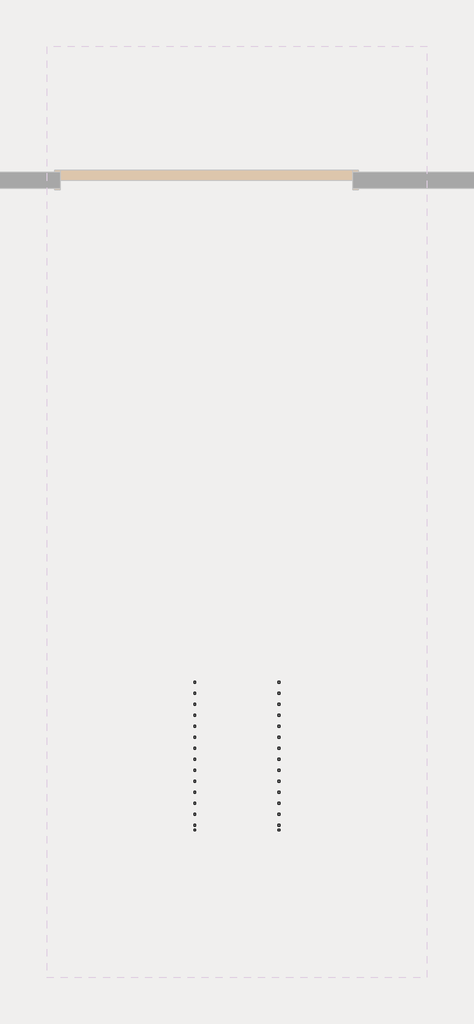
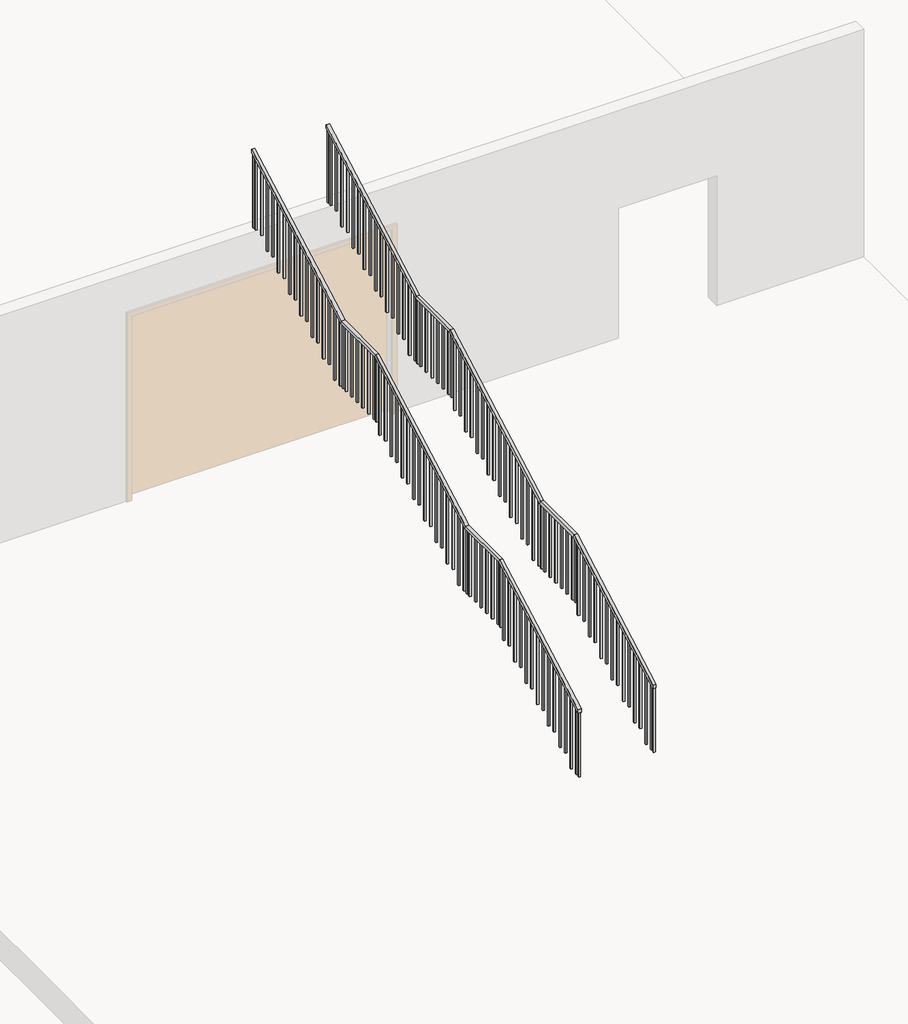
# One storey, part 9 of 13: 2 railings.
"""IFC4 building model written with IfcOpenShell, lengths in millimetres."""

from ifc_helpers import new_model, si_unit, frame, origin, place, context, project, spatial, polyline, outline, extrude, faceted_brep, element, save

model = new_model("IFC4")

# Units and contexts
model_context = context("Model", 3, world=origin())
ifc_project = project(units=[si_unit("LENGTHUNIT", "METRE", prefix="MILLI")], contexts=[model_context])

# Site, building, storey
site = spatial("IfcSite", under=ifc_project)
building = spatial("IfcBuilding", under=site)
storey = spatial("IfcBuildingStorey", under=building, Name="L0 - Ground Floor (Shadows On)", Elevation=0.0)

# Railings
placement = place(None, origin())
element("IfcRailing", 1, ObjectType="1100mm", at=placement, inside=storey, context=model_context, shape_type="SolidModel", body=[
    faceted_brep([(20443.6510627, -13941.7341454, 1266.6666667), (20443.6510627, -13941.7341454, 1209.4687214), (20493.6510627, -13941.7341454, 1209.4687214), (20493.6510627, -13941.7341454, 1266.6666667), (20443.6510627, -11841.7341454, 2433.3333333), (20443.6510627, -11828.7778439, 2383.3333333), (20493.6510627, -11828.7778439, 2383.3333333), (20493.6510627, -11841.7341454, 2433.3333333), (20443.6510627, -10941.7341454, 2433.3333333), (20443.6510627, -10928.7778439, 2383.3333333), (20493.6510627, -10928.7778439, 2383.3333333), (20493.6510627, -10941.7341454, 2433.3333333), (20443.6510627, -8541.7341454, 3766.6666667), (20443.6510627, -8528.7778439, 3716.6666667), (20493.6510627, -8528.7778439, 3716.6666667), (20493.6510627, -8541.7341454, 3766.6666667), (20443.6510627, -7641.7341454, 3766.6666667), (20443.6510627, -7628.7778439, 3716.6666667), (20493.6510627, -7628.7778439, 3716.6666667), (20493.6510627, -7641.7341454, 3766.6666667), (20443.6510627, -5241.7341454, 5100.0), (20493.6510627, -5241.7341454, 5100.0), (20493.6510627, -5241.7341454, 5042.8020548), (20443.6510627, -5241.7341454, 5042.8020548)], [[[0, 1, 2, 3]], [[1, 0, 4, 5]], [[2, 1, 5, 6]], [[3, 2, 6, 7]], [[0, 3, 7, 4]], [[5, 4, 8, 9]], [[6, 5, 9, 10]], [[7, 6, 10, 11]], [[4, 7, 11, 8]], [[9, 8, 12, 13]], [[10, 9, 13, 14]], [[11, 10, 14, 15]], [[8, 11, 15, 12]], [[13, 12, 16, 17]], [[14, 13, 17, 18]], [[15, 14, 18, 19]], [[12, 15, 19, 16]], [[20, 21, 22, 23]], [[17, 16, 20, 23]], [[18, 17, 23, 22]], [[19, 18, 22, 21]], [[16, 19, 21, 20]]]),
    extrude(outline(polyline([(-5329.2341454, 3833.3333333), (-5329.2341454, 4994.1909437), (-5304.2341454, 5008.0798326), (-5304.2341454, 3833.3333333), (-5329.2341454, 3833.3333333)])), frame((20456.1510627, 0.0, 0.0), z_axis=(1.0, 0.0, 0.0), x_axis=(0.0, 1.0, 0.0)), (0.0, 0.0, 1.0), 25.0),
    extrude(outline(polyline([(-5479.2341454, 3833.3333333), (-5479.2341454, 4910.8576103), (-5454.2341454, 4924.7464992), (-5454.2341454, 3833.3333333), (-5479.2341454, 3833.3333333)])), frame((20456.1510627, 0.0, 0.0), z_axis=(1.0, 0.0, 0.0), x_axis=(0.0, 1.0, 0.0)), (0.0, 0.0, 1.0), 25.0),
    extrude(outline(polyline([(-5629.2341454, 3666.6666667), (-5629.2341454, 4827.524277), (-5604.2341454, 4841.4131659), (-5604.2341454, 3666.6666667), (-5629.2341454, 3666.6666667)])), frame((20456.1510627, 0.0, 0.0), z_axis=(1.0, 0.0, 0.0), x_axis=(0.0, 1.0, 0.0)), (0.0, 0.0, 1.0), 25.0),
    extrude(outline(polyline([(-5779.2341454, 3666.6666667), (-5779.2341454, 4744.1909437), (-5754.2341454, 4758.0798326), (-5754.2341454, 3666.6666667), (-5779.2341454, 3666.6666667)])), frame((20456.1510627, 0.0, 0.0), z_axis=(1.0, 0.0, 0.0), x_axis=(0.0, 1.0, 0.0)), (0.0, 0.0, 1.0), 25.0),
    extrude(outline(polyline([(-5929.2341454, 3500.0), (-5929.2341454, 4660.8576103), (-5904.2341454, 4674.7464992), (-5904.2341454, 3500.0), (-5929.2341454, 3500.0)])), frame((20456.1510627, 0.0, 0.0), z_axis=(1.0, 0.0, 0.0), x_axis=(0.0, 1.0, 0.0)), (0.0, 0.0, 1.0), 25.0),
    extrude(outline(polyline([(-6079.2341454, 3500.0), (-6079.2341454, 4577.524277), (-6054.2341454, 4591.4131659), (-6054.2341454, 3500.0), (-6079.2341454, 3500.0)])), frame((20456.1510627, 0.0, 0.0), z_axis=(1.0, 0.0, 0.0), x_axis=(0.0, 1.0, 0.0)), (0.0, 0.0, 1.0), 25.0),
    extrude(outline(polyline([(-6229.2341454, 3333.3333333), (-6229.2341454, 4494.1909437), (-6204.2341454, 4508.0798326), (-6204.2341454, 3333.3333333), (-6229.2341454, 3333.3333333)])), frame((20456.1510627, 0.0, 0.0), z_axis=(1.0, 0.0, 0.0), x_axis=(0.0, 1.0, 0.0)), (0.0, 0.0, 1.0), 25.0),
    extrude(outline(polyline([(-6379.2341454, 3333.3333333), (-6379.2341454, 4410.8576103), (-6354.2341454, 4424.7464992), (-6354.2341454, 3333.3333333), (-6379.2341454, 3333.3333333)])), frame((20456.1510627, 0.0, 0.0), z_axis=(1.0, 0.0, 0.0), x_axis=(0.0, 1.0, 0.0)), (0.0, 0.0, 1.0), 25.0),
    extrude(outline(polyline([(-6529.2341454, 3166.6666667), (-6529.2341454, 4327.524277), (-6504.2341454, 4341.4131659), (-6504.2341454, 3166.6666667), (-6529.2341454, 3166.6666667)])), frame((20456.1510627, 0.0, 0.0), z_axis=(1.0, 0.0, 0.0), x_axis=(0.0, 1.0, 0.0)), (0.0, 0.0, 1.0), 25.0),
    extrude(outline(polyline([(-6679.2341454, 3166.6666667), (-6679.2341454, 4244.1909437), (-6654.2341454, 4258.0798326), (-6654.2341454, 3166.6666667), (-6679.2341454, 3166.6666667)])), frame((20456.1510627, 0.0, 0.0), z_axis=(1.0, 0.0, 0.0), x_axis=(0.0, 1.0, 0.0)), (0.0, 0.0, 1.0), 25.0),
    extrude(outline(polyline([(-6829.2341454, 3000.0), (-6829.2341454, 4160.8576103), (-6804.2341454, 4174.7464992), (-6804.2341454, 3000.0), (-6829.2341454, 3000.0)])), frame((20456.1510627, 0.0, 0.0), z_axis=(1.0, 0.0, 0.0), x_axis=(0.0, 1.0, 0.0)), (0.0, 0.0, 1.0), 25.0),
    extrude(outline(polyline([(-6979.2341454, 3000.0), (-6979.2341454, 4077.524277), (-6954.2341454, 4091.4131659), (-6954.2341454, 3000.0), (-6979.2341454, 3000.0)])), frame((20456.1510627, 0.0, 0.0), z_axis=(1.0, 0.0, 0.0), x_axis=(0.0, 1.0, 0.0)), (0.0, 0.0, 1.0), 25.0),
    extrude(outline(polyline([(-7129.2341454, 2833.3333333), (-7129.2341454, 3994.1909437), (-7104.2341454, 4008.0798326), (-7104.2341454, 2833.3333333), (-7129.2341454, 2833.3333333)])), frame((20456.1510627, 0.0, 0.0), z_axis=(1.0, 0.0, 0.0), x_axis=(0.0, 1.0, 0.0)), (0.0, 0.0, 1.0), 25.0),
    extrude(outline(polyline([(-7279.2341454, 2833.3333333), (-7279.2341454, 3910.8576103), (-7254.2341454, 3924.7464992), (-7254.2341454, 2833.3333333), (-7279.2341454, 2833.3333333)])), frame((20456.1510627, 0.0, 0.0), z_axis=(1.0, 0.0, 0.0), x_axis=(0.0, 1.0, 0.0)), (0.0, 0.0, 1.0), 25.0),
    extrude(outline(polyline([(-7429.2341454, 2666.6666667), (-7429.2341454, 3827.524277), (-7404.2341454, 3841.4131659), (-7404.2341454, 2666.6666667), (-7429.2341454, 2666.6666667)])), frame((20456.1510627, 0.0, 0.0), z_axis=(1.0, 0.0, 0.0), x_axis=(0.0, 1.0, 0.0)), (0.0, 0.0, 1.0), 25.0),
    extrude(outline(polyline([(-7579.2341454, 2666.6666667), (-7579.2341454, 3744.1909437), (-7554.2341454, 3758.0798326), (-7554.2341454, 2666.6666667), (-7579.2341454, 2666.6666667)])), frame((20456.1510627, 0.0, 0.0), z_axis=(1.0, 0.0, 0.0), x_axis=(0.0, 1.0, 0.0)), (0.0, 0.0, 1.0), 25.0),
    extrude(outline(polyline([(20481.1510627, -7729.2341454), (20456.1510627, -7729.2341454), (20456.1510627, -7704.2341454), (20481.1510627, -7704.2341454), (20481.1510627, -7729.2341454)])), frame((0.0, 0.0, 2666.6666667), z_axis=(0.0, 0.0, 1.0), x_axis=(1.0, 0.0, 0.0)), (0.0, 0.0, 1.0), 1050.0),
    extrude(outline(polyline([(20481.1510627, -7879.2341454), (20456.1510627, -7879.2341454), (20456.1510627, -7854.2341454), (20481.1510627, -7854.2341454), (20481.1510627, -7879.2341454)])), frame((0.0, 0.0, 2666.6666667), z_axis=(0.0, 0.0, 1.0), x_axis=(1.0, 0.0, 0.0)), (0.0, 0.0, 1.0), 1050.0),
    extrude(outline(polyline([(20481.1510627, -8029.2341454), (20456.1510627, -8029.2341454), (20456.1510627, -8004.2341454), (20481.1510627, -8004.2341454), (20481.1510627, -8029.2341454)])), frame((0.0, 0.0, 2666.6666667), z_axis=(0.0, 0.0, 1.0), x_axis=(1.0, 0.0, 0.0)), (0.0, 0.0, 1.0), 1050.0),
    extrude(outline(polyline([(20481.1510627, -8179.2341454), (20456.1510627, -8179.2341454), (20456.1510627, -8154.2341454), (20481.1510627, -8154.2341454), (20481.1510627, -8179.2341454)])), frame((0.0, 0.0, 2666.6666667), z_axis=(0.0, 0.0, 1.0), x_axis=(1.0, 0.0, 0.0)), (0.0, 0.0, 1.0), 1050.0),
    extrude(outline(polyline([(20481.1510627, -8329.2341454), (20456.1510627, -8329.2341454), (20456.1510627, -8304.2341454), (20481.1510627, -8304.2341454), (20481.1510627, -8329.2341454)])), frame((0.0, 0.0, 2666.6666667), z_axis=(0.0, 0.0, 1.0), x_axis=(1.0, 0.0, 0.0)), (0.0, 0.0, 1.0), 1050.0),
    extrude(outline(polyline([(20481.1510627, -8479.2341454), (20456.1510627, -8479.2341454), (20456.1510627, -8454.2341454), (20481.1510627, -8454.2341454), (20481.1510627, -8479.2341454)])), frame((0.0, 0.0, 2666.6666667), z_axis=(0.0, 0.0, 1.0), x_axis=(1.0, 0.0, 0.0)), (0.0, 0.0, 1.0), 1050.0),
    extrude(outline(polyline([(-8629.2341454, 2500.0), (-8629.2341454, 3660.8576103), (-8604.2341454, 3674.7464992), (-8604.2341454, 2500.0), (-8629.2341454, 2500.0)])), frame((20456.1510627, 0.0, 0.0), z_axis=(1.0, 0.0, 0.0), x_axis=(0.0, 1.0, 0.0)), (0.0, 0.0, 1.0), 25.0),
    extrude(outline(polyline([(-8779.2341454, 2500.0), (-8779.2341454, 3577.524277), (-8754.2341454, 3591.4131659), (-8754.2341454, 2500.0), (-8779.2341454, 2500.0)])), frame((20456.1510627, 0.0, 0.0), z_axis=(1.0, 0.0, 0.0), x_axis=(0.0, 1.0, 0.0)), (0.0, 0.0, 1.0), 25.0),
    extrude(outline(polyline([(-8929.2341454, 2333.3333333), (-8929.2341454, 3494.1909437), (-8904.2341454, 3508.0798326), (-8904.2341454, 2333.3333333), (-8929.2341454, 2333.3333333)])), frame((20456.1510627, 0.0, 0.0), z_axis=(1.0, 0.0, 0.0), x_axis=(0.0, 1.0, 0.0)), (0.0, 0.0, 1.0), 25.0),
    extrude(outline(polyline([(-9079.2341454, 2333.3333333), (-9079.2341454, 3410.8576103), (-9054.2341454, 3424.7464992), (-9054.2341454, 2333.3333333), (-9079.2341454, 2333.3333333)])), frame((20456.1510627, 0.0, 0.0), z_axis=(1.0, 0.0, 0.0), x_axis=(0.0, 1.0, 0.0)), (0.0, 0.0, 1.0), 25.0),
    extrude(outline(polyline([(-9229.2341454, 2166.6666667), (-9229.2341454, 3327.524277), (-9204.2341454, 3341.4131659), (-9204.2341454, 2166.6666667), (-9229.2341454, 2166.6666667)])), frame((20456.1510627, 0.0, 0.0), z_axis=(1.0, 0.0, 0.0), x_axis=(0.0, 1.0, 0.0)), (0.0, 0.0, 1.0), 25.0),
    extrude(outline(polyline([(-9379.2341454, 2166.6666667), (-9379.2341454, 3244.1909437), (-9354.2341454, 3258.0798326), (-9354.2341454, 2166.6666667), (-9379.2341454, 2166.6666667)])), frame((20456.1510627, 0.0, 0.0), z_axis=(1.0, 0.0, 0.0), x_axis=(0.0, 1.0, 0.0)), (0.0, 0.0, 1.0), 25.0),
    extrude(outline(polyline([(-9529.2341454, 2000.0), (-9529.2341454, 3160.8576103), (-9504.2341454, 3174.7464992), (-9504.2341454, 2000.0), (-9529.2341454, 2000.0)])), frame((20456.1510627, 0.0, 0.0), z_axis=(1.0, 0.0, 0.0), x_axis=(0.0, 1.0, 0.0)), (0.0, 0.0, 1.0), 25.0),
    extrude(outline(polyline([(-9679.2341454, 2000.0), (-9679.2341454, 3077.524277), (-9654.2341454, 3091.4131659), (-9654.2341454, 2000.0), (-9679.2341454, 2000.0)])), frame((20456.1510627, 0.0, 0.0), z_axis=(1.0, 0.0, 0.0), x_axis=(0.0, 1.0, 0.0)), (0.0, 0.0, 1.0), 25.0),
    extrude(outline(polyline([(-9829.2341454, 1833.3333333), (-9829.2341454, 2994.1909437), (-9804.2341454, 3008.0798326), (-9804.2341454, 1833.3333333), (-9829.2341454, 1833.3333333)])), frame((20456.1510627, 0.0, 0.0), z_axis=(1.0, 0.0, 0.0), x_axis=(0.0, 1.0, 0.0)), (0.0, 0.0, 1.0), 25.0),
    extrude(outline(polyline([(-9979.2341454, 1833.3333333), (-9979.2341454, 2910.8576103), (-9954.2341454, 2924.7464992), (-9954.2341454, 1833.3333333), (-9979.2341454, 1833.3333333)])), frame((20456.1510627, 0.0, 0.0), z_axis=(1.0, 0.0, 0.0), x_axis=(0.0, 1.0, 0.0)), (0.0, 0.0, 1.0), 25.0),
    extrude(outline(polyline([(-10129.2341454, 1666.6666667), (-10129.2341454, 2827.524277), (-10104.2341454, 2841.4131659), (-10104.2341454, 1666.6666667), (-10129.2341454, 1666.6666667)])), frame((20456.1510627, 0.0, 0.0), z_axis=(1.0, 0.0, 0.0), x_axis=(0.0, 1.0, 0.0)), (0.0, 0.0, 1.0), 25.0),
    extrude(outline(polyline([(-10279.2341454, 1666.6666667), (-10279.2341454, 2744.1909437), (-10254.2341454, 2758.0798326), (-10254.2341454, 1666.6666667), (-10279.2341454, 1666.6666667)])), frame((20456.1510627, 0.0, 0.0), z_axis=(1.0, 0.0, 0.0), x_axis=(0.0, 1.0, 0.0)), (0.0, 0.0, 1.0), 25.0),
    extrude(outline(polyline([(-10429.2341454, 1500.0), (-10429.2341454, 2660.8576103), (-10404.2341454, 2674.7464992), (-10404.2341454, 1500.0), (-10429.2341454, 1500.0)])), frame((20456.1510627, 0.0, 0.0), z_axis=(1.0, 0.0, 0.0), x_axis=(0.0, 1.0, 0.0)), (0.0, 0.0, 1.0), 25.0),
    extrude(outline(polyline([(-10579.2341454, 1500.0), (-10579.2341454, 2577.524277), (-10554.2341454, 2591.4131659), (-10554.2341454, 1500.0), (-10579.2341454, 1500.0)])), frame((20456.1510627, 0.0, 0.0), z_axis=(1.0, 0.0, 0.0), x_axis=(0.0, 1.0, 0.0)), (0.0, 0.0, 1.0), 25.0),
    extrude(outline(polyline([(-10729.2341454, 1333.3333333), (-10729.2341454, 2494.1909437), (-10704.2341454, 2508.0798326), (-10704.2341454, 1333.3333333), (-10729.2341454, 1333.3333333)])), frame((20456.1510627, 0.0, 0.0), z_axis=(1.0, 0.0, 0.0), x_axis=(0.0, 1.0, 0.0)), (0.0, 0.0, 1.0), 25.0),
    extrude(outline(polyline([(-10879.2341454, 1333.3333333), (-10879.2341454, 2410.8576103), (-10854.2341454, 2424.7464992), (-10854.2341454, 1333.3333333), (-10879.2341454, 1333.3333333)])), frame((20456.1510627, 0.0, 0.0), z_axis=(1.0, 0.0, 0.0), x_axis=(0.0, 1.0, 0.0)), (0.0, 0.0, 1.0), 25.0),
    extrude(outline(polyline([(20481.1510627, -11029.2341454), (20456.1510627, -11029.2341454), (20456.1510627, -11004.2341454), (20481.1510627, -11004.2341454), (20481.1510627, -11029.2341454)])), frame((0.0, 0.0, 1333.3333333), z_axis=(0.0, 0.0, 1.0), x_axis=(1.0, 0.0, 0.0)), (0.0, 0.0, 1.0), 1050.0),
    extrude(outline(polyline([(20481.1510627, -11179.2341454), (20456.1510627, -11179.2341454), (20456.1510627, -11154.2341454), (20481.1510627, -11154.2341454), (20481.1510627, -11179.2341454)])), frame((0.0, 0.0, 1333.3333333), z_axis=(0.0, 0.0, 1.0), x_axis=(1.0, 0.0, 0.0)), (0.0, 0.0, 1.0), 1050.0),
    extrude(outline(polyline([(20481.1510627, -11329.2341454), (20456.1510627, -11329.2341454), (20456.1510627, -11304.2341454), (20481.1510627, -11304.2341454), (20481.1510627, -11329.2341454)])), frame((0.0, 0.0, 1333.3333333), z_axis=(0.0, 0.0, 1.0), x_axis=(1.0, 0.0, 0.0)), (0.0, 0.0, 1.0), 1050.0),
    extrude(outline(polyline([(20481.1510627, -11479.2341454), (20456.1510627, -11479.2341454), (20456.1510627, -11454.2341454), (20481.1510627, -11454.2341454), (20481.1510627, -11479.2341454)])), frame((0.0, 0.0, 1333.3333333), z_axis=(0.0, 0.0, 1.0), x_axis=(1.0, 0.0, 0.0)), (0.0, 0.0, 1.0), 1050.0),
    extrude(outline(polyline([(20481.1510627, -11629.2341454), (20456.1510627, -11629.2341454), (20456.1510627, -11604.2341454), (20481.1510627, -11604.2341454), (20481.1510627, -11629.2341454)])), frame((0.0, 0.0, 1333.3333333), z_axis=(0.0, 0.0, 1.0), x_axis=(1.0, 0.0, 0.0)), (0.0, 0.0, 1.0), 1050.0),
    extrude(outline(polyline([(20481.1510627, -11779.2341454), (20456.1510627, -11779.2341454), (20456.1510627, -11754.2341454), (20481.1510627, -11754.2341454), (20481.1510627, -11779.2341454)])), frame((0.0, 0.0, 1333.3333333), z_axis=(0.0, 0.0, 1.0), x_axis=(1.0, 0.0, 0.0)), (0.0, 0.0, 1.0), 1050.0),
    extrude(outline(polyline([(-11929.2341454, 1166.6666667), (-11929.2341454, 2327.524277), (-11904.2341454, 2341.4131659), (-11904.2341454, 1166.6666667), (-11929.2341454, 1166.6666667)])), frame((20456.1510627, 0.0, 0.0), z_axis=(1.0, 0.0, 0.0), x_axis=(0.0, 1.0, 0.0)), (0.0, 0.0, 1.0), 25.0),
    extrude(outline(polyline([(-12079.2341454, 1166.6666667), (-12079.2341454, 2244.1909437), (-12054.2341454, 2258.0798326), (-12054.2341454, 1166.6666667), (-12079.2341454, 1166.6666667)])), frame((20456.1510627, 0.0, 0.0), z_axis=(1.0, 0.0, 0.0), x_axis=(0.0, 1.0, 0.0)), (0.0, 0.0, 1.0), 25.0),
    extrude(outline(polyline([(-12229.2341454, 1000.0), (-12229.2341454, 2160.8576103), (-12204.2341454, 2174.7464992), (-12204.2341454, 1000.0), (-12229.2341454, 1000.0)])), frame((20456.1510627, 0.0, 0.0), z_axis=(1.0, 0.0, 0.0), x_axis=(0.0, 1.0, 0.0)), (0.0, 0.0, 1.0), 25.0),
    extrude(outline(polyline([(-12379.2341454, 1000.0), (-12379.2341454, 2077.524277), (-12354.2341454, 2091.4131659), (-12354.2341454, 1000.0), (-12379.2341454, 1000.0)])), frame((20456.1510627, 0.0, 0.0), z_axis=(1.0, 0.0, 0.0), x_axis=(0.0, 1.0, 0.0)), (0.0, 0.0, 1.0), 25.0),
    extrude(outline(polyline([(-12529.2341454, 833.3333333), (-12529.2341454, 1994.1909437), (-12504.2341454, 2008.0798326), (-12504.2341454, 833.3333333), (-12529.2341454, 833.3333333)])), frame((20456.1510627, 0.0, 0.0), z_axis=(1.0, 0.0, 0.0), x_axis=(0.0, 1.0, 0.0)), (0.0, 0.0, 1.0), 25.0),
    extrude(outline(polyline([(-12679.2341454, 833.3333333), (-12679.2341454, 1910.8576103), (-12654.2341454, 1924.7464992), (-12654.2341454, 833.3333333), (-12679.2341454, 833.3333333)])), frame((20456.1510627, 0.0, 0.0), z_axis=(1.0, 0.0, 0.0), x_axis=(0.0, 1.0, 0.0)), (0.0, 0.0, 1.0), 25.0),
    extrude(outline(polyline([(-12829.2341454, 666.6666667), (-12829.2341454, 1827.524277), (-12804.2341454, 1841.4131659), (-12804.2341454, 666.6666667), (-12829.2341454, 666.6666667)])), frame((20456.1510627, 0.0, 0.0), z_axis=(1.0, 0.0, 0.0), x_axis=(0.0, 1.0, 0.0)), (0.0, 0.0, 1.0), 25.0),
    extrude(outline(polyline([(-12979.2341454, 666.6666667), (-12979.2341454, 1744.1909437), (-12954.2341454, 1758.0798326), (-12954.2341454, 666.6666667), (-12979.2341454, 666.6666667)])), frame((20456.1510627, 0.0, 0.0), z_axis=(1.0, 0.0, 0.0), x_axis=(0.0, 1.0, 0.0)), (0.0, 0.0, 1.0), 25.0),
    extrude(outline(polyline([(-13129.2341454, 500.0), (-13129.2341454, 1660.8576103), (-13104.2341454, 1674.7464992), (-13104.2341454, 500.0), (-13129.2341454, 500.0)])), frame((20456.1510627, 0.0, 0.0), z_axis=(1.0, 0.0, 0.0), x_axis=(0.0, 1.0, 0.0)), (0.0, 0.0, 1.0), 25.0),
    extrude(outline(polyline([(-13279.2341454, 500.0), (-13279.2341454, 1577.524277), (-13254.2341454, 1591.4131659), (-13254.2341454, 500.0), (-13279.2341454, 500.0)])), frame((20456.1510627, 0.0, 0.0), z_axis=(1.0, 0.0, 0.0), x_axis=(0.0, 1.0, 0.0)), (0.0, 0.0, 1.0), 25.0),
    extrude(outline(polyline([(-13429.2341454, 333.3333333), (-13429.2341454, 1494.1909437), (-13404.2341454, 1508.0798326), (-13404.2341454, 333.3333333), (-13429.2341454, 333.3333333)])), frame((20456.1510627, 0.0, 0.0), z_axis=(1.0, 0.0, 0.0), x_axis=(0.0, 1.0, 0.0)), (0.0, 0.0, 1.0), 25.0),
    extrude(outline(polyline([(-13579.2341454, 333.3333333), (-13579.2341454, 1410.8576103), (-13554.2341454, 1424.7464992), (-13554.2341454, 333.3333333), (-13579.2341454, 333.3333333)])), frame((20456.1510627, 0.0, 0.0), z_axis=(1.0, 0.0, 0.0), x_axis=(0.0, 1.0, 0.0)), (0.0, 0.0, 1.0), 25.0),
    extrude(outline(polyline([(-13729.2341454, 166.6666667), (-13729.2341454, 1327.524277), (-13704.2341454, 1341.4131659), (-13704.2341454, 166.6666667), (-13729.2341454, 166.6666667)])), frame((20456.1510627, 0.0, 0.0), z_axis=(1.0, 0.0, 0.0), x_axis=(0.0, 1.0, 0.0)), (0.0, 0.0, 1.0), 25.0),
    extrude(outline(polyline([(-13879.2341454, 166.6666667), (-13879.2341454, 1244.1909437), (-13854.2341454, 1258.0798326), (-13854.2341454, 166.6666667), (-13879.2341454, 166.6666667)])), frame((20456.1510627, 0.0, 0.0), z_axis=(1.0, 0.0, 0.0), x_axis=(0.0, 1.0, 0.0)), (0.0, 0.0, 1.0), 25.0),
    extrude(outline(polyline([(20481.1510627, -7654.2341454), (20456.1510627, -7654.2341454), (20456.1510627, -7629.2341454), (20481.1510627, -7629.2341454), (20481.1510627, -7654.2341454)])), frame((0.0, 0.0, 2666.6666667), z_axis=(0.0, 0.0, 1.0), x_axis=(1.0, 0.0, 0.0)), (0.0, 0.0, 1.0), 1050.0),
    extrude(outline(polyline([(-8554.2341454, 2666.6666667), (-8554.2341454, 3702.524277), (-8529.2341454, 3716.4131659), (-8529.2341454, 2666.6666667), (-8554.2341454, 2666.6666667)])), frame((20456.1510627, 0.0, 0.0), z_axis=(1.0, 0.0, 0.0), x_axis=(0.0, 1.0, 0.0)), (0.0, 0.0, 1.0), 25.0),
    extrude(outline(polyline([(20481.1510627, -10954.2341454), (20456.1510627, -10954.2341454), (20456.1510627, -10929.2341454), (20481.1510627, -10929.2341454), (20481.1510627, -10954.2341454)])), frame((0.0, 0.0, 1333.3333333), z_axis=(0.0, 0.0, 1.0), x_axis=(1.0, 0.0, 0.0)), (0.0, 0.0, 1.0), 1050.0),
    extrude(outline(polyline([(-11854.2341454, 1333.3333333), (-11854.2341454, 2369.1909437), (-11829.2341454, 2383.0798326), (-11829.2341454, 1333.3333333), (-11854.2341454, 1333.3333333)])), frame((20456.1510627, 0.0, 0.0), z_axis=(1.0, 0.0, 0.0), x_axis=(0.0, 1.0, 0.0)), (0.0, 0.0, 1.0), 25.0),
    extrude(outline(polyline([(-5266.7341454, 3833.3333333), (-5266.7341454, 5028.9131659), (-5241.7341454, 5042.8020548), (-5241.7341454, 3833.3333333), (-5266.7341454, 3833.3333333)])), frame((20456.1510627, 0.0, 0.0), z_axis=(1.0, 0.0, 0.0), x_axis=(0.0, 1.0, 0.0)), (0.0, 0.0, 1.0), 25.0),
    extrude(outline(polyline([(-13941.7341454, 166.6666667), (-13941.7341454, 1209.4687214), (-13916.7341454, 1223.3576103), (-13916.7341454, 166.6666667), (-13941.7341454, 166.6666667)])), frame((20456.1510627, 0.0, 0.0), z_axis=(1.0, 0.0, 0.0), x_axis=(0.0, 1.0, 0.0)), (0.0, 0.0, 1.0), 25.0),
])
element("IfcRailing", 2, ObjectType="1100mm", at=placement, inside=storey, context=model_context, shape_type="SolidModel", body=[
    faceted_brep([(19294.4510627, -13941.7341454, 1266.6666667), (19294.4510627, -13941.7341454, 1209.4687214), (19344.4510627, -13941.7341454, 1209.4687214), (19344.4510627, -13941.7341454, 1266.6666667), (19294.4510627, -11841.7341454, 2433.3333333), (19294.4510627, -11828.7778439, 2383.3333333), (19344.4510627, -11828.7778439, 2383.3333333), (19344.4510627, -11841.7341454, 2433.3333333), (19294.4510627, -10941.7341454, 2433.3333333), (19294.4510627, -10928.7778439, 2383.3333333), (19344.4510627, -10928.7778439, 2383.3333333), (19344.4510627, -10941.7341454, 2433.3333333), (19294.4510627, -8541.7341454, 3766.6666667), (19294.4510627, -8528.7778439, 3716.6666667), (19344.4510627, -8528.7778439, 3716.6666667), (19344.4510627, -8541.7341454, 3766.6666667), (19294.4510627, -7641.7341454, 3766.6666667), (19294.4510627, -7628.7778439, 3716.6666667), (19344.4510627, -7628.7778439, 3716.6666667), (19344.4510627, -7641.7341454, 3766.6666667), (19294.4510627, -5241.7341454, 5100.0), (19344.4510627, -5241.7341454, 5100.0), (19344.4510627, -5241.7341454, 5042.8020548), (19294.4510627, -5241.7341454, 5042.8020548)], [[[0, 1, 2, 3]], [[1, 0, 4, 5]], [[2, 1, 5, 6]], [[3, 2, 6, 7]], [[0, 3, 7, 4]], [[5, 4, 8, 9]], [[6, 5, 9, 10]], [[7, 6, 10, 11]], [[4, 7, 11, 8]], [[9, 8, 12, 13]], [[10, 9, 13, 14]], [[11, 10, 14, 15]], [[8, 11, 15, 12]], [[13, 12, 16, 17]], [[14, 13, 17, 18]], [[15, 14, 18, 19]], [[12, 15, 19, 16]], [[20, 21, 22, 23]], [[17, 16, 20, 23]], [[18, 17, 23, 22]], [[19, 18, 22, 21]], [[16, 19, 21, 20]]]),
    extrude(outline(polyline([(-5329.2341454, 4994.1909437), (-5304.2341454, 5008.0798326), (-5304.2341454, 3833.3333333), (-5329.2341454, 3833.3333333), (-5329.2341454, 4994.1909437)])), frame((19306.9510627, 0.0, 0.0), z_axis=(1.0, 0.0, 0.0), x_axis=(0.0, 1.0, 0.0)), (0.0, 0.0, 1.0), 25.0),
    extrude(outline(polyline([(-5479.2341454, 4910.8576103), (-5454.2341454, 4924.7464992), (-5454.2341454, 3833.3333333), (-5479.2341454, 3833.3333333), (-5479.2341454, 4910.8576103)])), frame((19306.9510627, 0.0, 0.0), z_axis=(1.0, 0.0, 0.0), x_axis=(0.0, 1.0, 0.0)), (0.0, 0.0, 1.0), 25.0),
    extrude(outline(polyline([(-5629.2341454, 4827.524277), (-5604.2341454, 4841.4131659), (-5604.2341454, 3666.6666667), (-5629.2341454, 3666.6666667), (-5629.2341454, 4827.524277)])), frame((19306.9510627, 0.0, 0.0), z_axis=(1.0, 0.0, 0.0), x_axis=(0.0, 1.0, 0.0)), (0.0, 0.0, 1.0), 25.0),
    extrude(outline(polyline([(-5779.2341454, 4744.1909437), (-5754.2341454, 4758.0798326), (-5754.2341454, 3666.6666667), (-5779.2341454, 3666.6666667), (-5779.2341454, 4744.1909437)])), frame((19306.9510627, 0.0, 0.0), z_axis=(1.0, 0.0, 0.0), x_axis=(0.0, 1.0, 0.0)), (0.0, 0.0, 1.0), 25.0),
    extrude(outline(polyline([(-5929.2341454, 4660.8576103), (-5904.2341454, 4674.7464992), (-5904.2341454, 3500.0), (-5929.2341454, 3500.0), (-5929.2341454, 4660.8576103)])), frame((19306.9510627, 0.0, 0.0), z_axis=(1.0, 0.0, 0.0), x_axis=(0.0, 1.0, 0.0)), (0.0, 0.0, 1.0), 25.0),
    extrude(outline(polyline([(-6079.2341454, 4577.524277), (-6054.2341454, 4591.4131659), (-6054.2341454, 3500.0), (-6079.2341454, 3500.0), (-6079.2341454, 4577.524277)])), frame((19306.9510627, 0.0, 0.0), z_axis=(1.0, 0.0, 0.0), x_axis=(0.0, 1.0, 0.0)), (0.0, 0.0, 1.0), 25.0),
    extrude(outline(polyline([(-6229.2341454, 4494.1909437), (-6204.2341454, 4508.0798326), (-6204.2341454, 3333.3333333), (-6229.2341454, 3333.3333333), (-6229.2341454, 4494.1909437)])), frame((19306.9510627, 0.0, 0.0), z_axis=(1.0, 0.0, 0.0), x_axis=(0.0, 1.0, 0.0)), (0.0, 0.0, 1.0), 25.0),
    extrude(outline(polyline([(-6379.2341454, 4410.8576103), (-6354.2341454, 4424.7464992), (-6354.2341454, 3333.3333333), (-6379.2341454, 3333.3333333), (-6379.2341454, 4410.8576103)])), frame((19306.9510627, 0.0, 0.0), z_axis=(1.0, 0.0, 0.0), x_axis=(0.0, 1.0, 0.0)), (0.0, 0.0, 1.0), 25.0),
    extrude(outline(polyline([(-6529.2341454, 4327.524277), (-6504.2341454, 4341.4131659), (-6504.2341454, 3166.6666667), (-6529.2341454, 3166.6666667), (-6529.2341454, 4327.524277)])), frame((19306.9510627, 0.0, 0.0), z_axis=(1.0, 0.0, 0.0), x_axis=(0.0, 1.0, 0.0)), (0.0, 0.0, 1.0), 25.0),
    extrude(outline(polyline([(-6679.2341454, 4244.1909437), (-6654.2341454, 4258.0798326), (-6654.2341454, 3166.6666667), (-6679.2341454, 3166.6666667), (-6679.2341454, 4244.1909437)])), frame((19306.9510627, 0.0, 0.0), z_axis=(1.0, 0.0, 0.0), x_axis=(0.0, 1.0, 0.0)), (0.0, 0.0, 1.0), 25.0),
    extrude(outline(polyline([(-6829.2341454, 4160.8576103), (-6804.2341454, 4174.7464992), (-6804.2341454, 3000.0), (-6829.2341454, 3000.0), (-6829.2341454, 4160.8576103)])), frame((19306.9510627, 0.0, 0.0), z_axis=(1.0, 0.0, 0.0), x_axis=(0.0, 1.0, 0.0)), (0.0, 0.0, 1.0), 25.0),
    extrude(outline(polyline([(-6979.2341454, 4077.524277), (-6954.2341454, 4091.4131659), (-6954.2341454, 3000.0), (-6979.2341454, 3000.0), (-6979.2341454, 4077.524277)])), frame((19306.9510627, 0.0, 0.0), z_axis=(1.0, 0.0, 0.0), x_axis=(0.0, 1.0, 0.0)), (0.0, 0.0, 1.0), 25.0),
    extrude(outline(polyline([(-7129.2341454, 3994.1909437), (-7104.2341454, 4008.0798326), (-7104.2341454, 2833.3333333), (-7129.2341454, 2833.3333333), (-7129.2341454, 3994.1909437)])), frame((19306.9510627, 0.0, 0.0), z_axis=(1.0, 0.0, 0.0), x_axis=(0.0, 1.0, 0.0)), (0.0, 0.0, 1.0), 25.0),
    extrude(outline(polyline([(-7279.2341454, 3910.8576103), (-7254.2341454, 3924.7464992), (-7254.2341454, 2833.3333333), (-7279.2341454, 2833.3333333), (-7279.2341454, 3910.8576103)])), frame((19306.9510627, 0.0, 0.0), z_axis=(1.0, 0.0, 0.0), x_axis=(0.0, 1.0, 0.0)), (0.0, 0.0, 1.0), 25.0),
    extrude(outline(polyline([(-7429.2341454, 3827.524277), (-7404.2341454, 3841.4131659), (-7404.2341454, 2666.6666667), (-7429.2341454, 2666.6666667), (-7429.2341454, 3827.524277)])), frame((19306.9510627, 0.0, 0.0), z_axis=(1.0, 0.0, 0.0), x_axis=(0.0, 1.0, 0.0)), (0.0, 0.0, 1.0), 25.0),
    extrude(outline(polyline([(-7579.2341454, 3744.1909437), (-7554.2341454, 3758.0798326), (-7554.2341454, 2666.6666667), (-7579.2341454, 2666.6666667), (-7579.2341454, 3744.1909437)])), frame((19306.9510627, 0.0, 0.0), z_axis=(1.0, 0.0, 0.0), x_axis=(0.0, 1.0, 0.0)), (0.0, 0.0, 1.0), 25.0),
    extrude(outline(polyline([(19306.9510627, -7729.2341454), (19306.9510627, -7704.2341454), (19331.9510627, -7704.2341454), (19331.9510627, -7729.2341454), (19306.9510627, -7729.2341454)])), frame((0.0, 0.0, 2666.6666667), z_axis=(0.0, 0.0, 1.0), x_axis=(1.0, 0.0, 0.0)), (0.0, 0.0, 1.0), 1050.0),
    extrude(outline(polyline([(19306.9510627, -7879.2341454), (19306.9510627, -7854.2341454), (19331.9510627, -7854.2341454), (19331.9510627, -7879.2341454), (19306.9510627, -7879.2341454)])), frame((0.0, 0.0, 2666.6666667), z_axis=(0.0, 0.0, 1.0), x_axis=(1.0, 0.0, 0.0)), (0.0, 0.0, 1.0), 1050.0),
    extrude(outline(polyline([(19306.9510627, -8029.2341454), (19306.9510627, -8004.2341454), (19331.9510627, -8004.2341454), (19331.9510627, -8029.2341454), (19306.9510627, -8029.2341454)])), frame((0.0, 0.0, 2666.6666667), z_axis=(0.0, 0.0, 1.0), x_axis=(1.0, 0.0, 0.0)), (0.0, 0.0, 1.0), 1050.0),
    extrude(outline(polyline([(19306.9510627, -8179.2341454), (19306.9510627, -8154.2341454), (19331.9510627, -8154.2341454), (19331.9510627, -8179.2341454), (19306.9510627, -8179.2341454)])), frame((0.0, 0.0, 2666.6666667), z_axis=(0.0, 0.0, 1.0), x_axis=(1.0, 0.0, 0.0)), (0.0, 0.0, 1.0), 1050.0),
    extrude(outline(polyline([(19306.9510627, -8329.2341454), (19306.9510627, -8304.2341454), (19331.9510627, -8304.2341454), (19331.9510627, -8329.2341454), (19306.9510627, -8329.2341454)])), frame((0.0, 0.0, 2666.6666667), z_axis=(0.0, 0.0, 1.0), x_axis=(1.0, 0.0, 0.0)), (0.0, 0.0, 1.0), 1050.0),
    extrude(outline(polyline([(19306.9510627, -8479.2341454), (19306.9510627, -8454.2341454), (19331.9510627, -8454.2341454), (19331.9510627, -8479.2341454), (19306.9510627, -8479.2341454)])), frame((0.0, 0.0, 2666.6666667), z_axis=(0.0, 0.0, 1.0), x_axis=(1.0, 0.0, 0.0)), (0.0, 0.0, 1.0), 1050.0),
    extrude(outline(polyline([(-8629.2341454, 3660.8576103), (-8604.2341454, 3674.7464992), (-8604.2341454, 2500.0), (-8629.2341454, 2500.0), (-8629.2341454, 3660.8576103)])), frame((19306.9510627, 0.0, 0.0), z_axis=(1.0, 0.0, 0.0), x_axis=(0.0, 1.0, 0.0)), (0.0, 0.0, 1.0), 25.0),
    extrude(outline(polyline([(-8779.2341454, 3577.524277), (-8754.2341454, 3591.4131659), (-8754.2341454, 2500.0), (-8779.2341454, 2500.0), (-8779.2341454, 3577.524277)])), frame((19306.9510627, 0.0, 0.0), z_axis=(1.0, 0.0, 0.0), x_axis=(0.0, 1.0, 0.0)), (0.0, 0.0, 1.0), 25.0),
    extrude(outline(polyline([(-8929.2341454, 3494.1909437), (-8904.2341454, 3508.0798326), (-8904.2341454, 2333.3333333), (-8929.2341454, 2333.3333333), (-8929.2341454, 3494.1909437)])), frame((19306.9510627, 0.0, 0.0), z_axis=(1.0, 0.0, 0.0), x_axis=(0.0, 1.0, 0.0)), (0.0, 0.0, 1.0), 25.0),
    extrude(outline(polyline([(-9079.2341454, 3410.8576103), (-9054.2341454, 3424.7464992), (-9054.2341454, 2333.3333333), (-9079.2341454, 2333.3333333), (-9079.2341454, 3410.8576103)])), frame((19306.9510627, 0.0, 0.0), z_axis=(1.0, 0.0, 0.0), x_axis=(0.0, 1.0, 0.0)), (0.0, 0.0, 1.0), 25.0),
    extrude(outline(polyline([(-9229.2341454, 3327.524277), (-9204.2341454, 3341.4131659), (-9204.2341454, 2166.6666667), (-9229.2341454, 2166.6666667), (-9229.2341454, 3327.524277)])), frame((19306.9510627, 0.0, 0.0), z_axis=(1.0, 0.0, 0.0), x_axis=(0.0, 1.0, 0.0)), (0.0, 0.0, 1.0), 25.0),
    extrude(outline(polyline([(-9379.2341454, 3244.1909437), (-9354.2341454, 3258.0798326), (-9354.2341454, 2166.6666667), (-9379.2341454, 2166.6666667), (-9379.2341454, 3244.1909437)])), frame((19306.9510627, 0.0, 0.0), z_axis=(1.0, 0.0, 0.0), x_axis=(0.0, 1.0, 0.0)), (0.0, 0.0, 1.0), 25.0),
    extrude(outline(polyline([(-9529.2341454, 3160.8576103), (-9504.2341454, 3174.7464992), (-9504.2341454, 2000.0), (-9529.2341454, 2000.0), (-9529.2341454, 3160.8576103)])), frame((19306.9510627, 0.0, 0.0), z_axis=(1.0, 0.0, 0.0), x_axis=(0.0, 1.0, 0.0)), (0.0, 0.0, 1.0), 25.0),
    extrude(outline(polyline([(-9679.2341454, 3077.524277), (-9654.2341454, 3091.4131659), (-9654.2341454, 2000.0), (-9679.2341454, 2000.0), (-9679.2341454, 3077.524277)])), frame((19306.9510627, 0.0, 0.0), z_axis=(1.0, 0.0, 0.0), x_axis=(0.0, 1.0, 0.0)), (0.0, 0.0, 1.0), 25.0),
    extrude(outline(polyline([(-9829.2341454, 2994.1909437), (-9804.2341454, 3008.0798326), (-9804.2341454, 1833.3333333), (-9829.2341454, 1833.3333333), (-9829.2341454, 2994.1909437)])), frame((19306.9510627, 0.0, 0.0), z_axis=(1.0, 0.0, 0.0), x_axis=(0.0, 1.0, 0.0)), (0.0, 0.0, 1.0), 25.0),
    extrude(outline(polyline([(-9979.2341454, 2910.8576103), (-9954.2341454, 2924.7464992), (-9954.2341454, 1833.3333333), (-9979.2341454, 1833.3333333), (-9979.2341454, 2910.8576103)])), frame((19306.9510627, 0.0, 0.0), z_axis=(1.0, 0.0, 0.0), x_axis=(0.0, 1.0, 0.0)), (0.0, 0.0, 1.0), 25.0),
    extrude(outline(polyline([(-10129.2341454, 2827.524277), (-10104.2341454, 2841.4131659), (-10104.2341454, 1666.6666667), (-10129.2341454, 1666.6666667), (-10129.2341454, 2827.524277)])), frame((19306.9510627, 0.0, 0.0), z_axis=(1.0, 0.0, 0.0), x_axis=(0.0, 1.0, 0.0)), (0.0, 0.0, 1.0), 25.0),
    extrude(outline(polyline([(-10279.2341454, 2744.1909437), (-10254.2341454, 2758.0798326), (-10254.2341454, 1666.6666667), (-10279.2341454, 1666.6666667), (-10279.2341454, 2744.1909437)])), frame((19306.9510627, 0.0, 0.0), z_axis=(1.0, 0.0, 0.0), x_axis=(0.0, 1.0, 0.0)), (0.0, 0.0, 1.0), 25.0),
    extrude(outline(polyline([(-10429.2341454, 2660.8576103), (-10404.2341454, 2674.7464992), (-10404.2341454, 1500.0), (-10429.2341454, 1500.0), (-10429.2341454, 2660.8576103)])), frame((19306.9510627, 0.0, 0.0), z_axis=(1.0, 0.0, 0.0), x_axis=(0.0, 1.0, 0.0)), (0.0, 0.0, 1.0), 25.0),
    extrude(outline(polyline([(-10579.2341454, 2577.524277), (-10554.2341454, 2591.4131659), (-10554.2341454, 1500.0), (-10579.2341454, 1500.0), (-10579.2341454, 2577.524277)])), frame((19306.9510627, 0.0, 0.0), z_axis=(1.0, 0.0, 0.0), x_axis=(0.0, 1.0, 0.0)), (0.0, 0.0, 1.0), 25.0),
    extrude(outline(polyline([(-10729.2341454, 2494.1909437), (-10704.2341454, 2508.0798326), (-10704.2341454, 1333.3333333), (-10729.2341454, 1333.3333333), (-10729.2341454, 2494.1909437)])), frame((19306.9510627, 0.0, 0.0), z_axis=(1.0, 0.0, 0.0), x_axis=(0.0, 1.0, 0.0)), (0.0, 0.0, 1.0), 25.0),
    extrude(outline(polyline([(-10879.2341454, 2410.8576103), (-10854.2341454, 2424.7464992), (-10854.2341454, 1333.3333333), (-10879.2341454, 1333.3333333), (-10879.2341454, 2410.8576103)])), frame((19306.9510627, 0.0, 0.0), z_axis=(1.0, 0.0, 0.0), x_axis=(0.0, 1.0, 0.0)), (0.0, 0.0, 1.0), 25.0),
    extrude(outline(polyline([(19306.9510627, -11029.2341454), (19306.9510627, -11004.2341454), (19331.9510627, -11004.2341454), (19331.9510627, -11029.2341454), (19306.9510627, -11029.2341454)])), frame((0.0, 0.0, 1333.3333333), z_axis=(0.0, 0.0, 1.0), x_axis=(1.0, 0.0, 0.0)), (0.0, 0.0, 1.0), 1050.0),
    extrude(outline(polyline([(19306.9510627, -11179.2341454), (19306.9510627, -11154.2341454), (19331.9510627, -11154.2341454), (19331.9510627, -11179.2341454), (19306.9510627, -11179.2341454)])), frame((0.0, 0.0, 1333.3333333), z_axis=(0.0, 0.0, 1.0), x_axis=(1.0, 0.0, 0.0)), (0.0, 0.0, 1.0), 1050.0),
    extrude(outline(polyline([(19306.9510627, -11329.2341454), (19306.9510627, -11304.2341454), (19331.9510627, -11304.2341454), (19331.9510627, -11329.2341454), (19306.9510627, -11329.2341454)])), frame((0.0, 0.0, 1333.3333333), z_axis=(0.0, 0.0, 1.0), x_axis=(1.0, 0.0, 0.0)), (0.0, 0.0, 1.0), 1050.0),
    extrude(outline(polyline([(19306.9510627, -11479.2341454), (19306.9510627, -11454.2341454), (19331.9510627, -11454.2341454), (19331.9510627, -11479.2341454), (19306.9510627, -11479.2341454)])), frame((0.0, 0.0, 1333.3333333), z_axis=(0.0, 0.0, 1.0), x_axis=(1.0, 0.0, 0.0)), (0.0, 0.0, 1.0), 1050.0),
    extrude(outline(polyline([(19306.9510627, -11629.2341454), (19306.9510627, -11604.2341454), (19331.9510627, -11604.2341454), (19331.9510627, -11629.2341454), (19306.9510627, -11629.2341454)])), frame((0.0, 0.0, 1333.3333333), z_axis=(0.0, 0.0, 1.0), x_axis=(1.0, 0.0, 0.0)), (0.0, 0.0, 1.0), 1050.0),
    extrude(outline(polyline([(19306.9510627, -11779.2341454), (19306.9510627, -11754.2341454), (19331.9510627, -11754.2341454), (19331.9510627, -11779.2341454), (19306.9510627, -11779.2341454)])), frame((0.0, 0.0, 1333.3333333), z_axis=(0.0, 0.0, 1.0), x_axis=(1.0, 0.0, 0.0)), (0.0, 0.0, 1.0), 1050.0),
    extrude(outline(polyline([(-11929.2341454, 2327.524277), (-11904.2341454, 2341.4131659), (-11904.2341454, 1166.6666667), (-11929.2341454, 1166.6666667), (-11929.2341454, 2327.524277)])), frame((19306.9510627, 0.0, 0.0), z_axis=(1.0, 0.0, 0.0), x_axis=(0.0, 1.0, 0.0)), (0.0, 0.0, 1.0), 25.0),
    extrude(outline(polyline([(-12079.2341454, 2244.1909437), (-12054.2341454, 2258.0798326), (-12054.2341454, 1166.6666667), (-12079.2341454, 1166.6666667), (-12079.2341454, 2244.1909437)])), frame((19306.9510627, 0.0, 0.0), z_axis=(1.0, 0.0, 0.0), x_axis=(0.0, 1.0, 0.0)), (0.0, 0.0, 1.0), 25.0),
    extrude(outline(polyline([(-12229.2341454, 2160.8576103), (-12204.2341454, 2174.7464992), (-12204.2341454, 1000.0), (-12229.2341454, 1000.0), (-12229.2341454, 2160.8576103)])), frame((19306.9510627, 0.0, 0.0), z_axis=(1.0, 0.0, 0.0), x_axis=(0.0, 1.0, 0.0)), (0.0, 0.0, 1.0), 25.0),
    extrude(outline(polyline([(-12379.2341454, 2077.524277), (-12354.2341454, 2091.4131659), (-12354.2341454, 1000.0), (-12379.2341454, 1000.0), (-12379.2341454, 2077.524277)])), frame((19306.9510627, 0.0, 0.0), z_axis=(1.0, 0.0, 0.0), x_axis=(0.0, 1.0, 0.0)), (0.0, 0.0, 1.0), 25.0),
    extrude(outline(polyline([(-12529.2341454, 1994.1909437), (-12504.2341454, 2008.0798326), (-12504.2341454, 833.3333333), (-12529.2341454, 833.3333333), (-12529.2341454, 1994.1909437)])), frame((19306.9510627, 0.0, 0.0), z_axis=(1.0, 0.0, 0.0), x_axis=(0.0, 1.0, 0.0)), (0.0, 0.0, 1.0), 25.0),
    extrude(outline(polyline([(-12679.2341454, 1910.8576103), (-12654.2341454, 1924.7464992), (-12654.2341454, 833.3333333), (-12679.2341454, 833.3333333), (-12679.2341454, 1910.8576103)])), frame((19306.9510627, 0.0, 0.0), z_axis=(1.0, 0.0, 0.0), x_axis=(0.0, 1.0, 0.0)), (0.0, 0.0, 1.0), 25.0),
    extrude(outline(polyline([(-12829.2341454, 1827.524277), (-12804.2341454, 1841.4131659), (-12804.2341454, 666.6666667), (-12829.2341454, 666.6666667), (-12829.2341454, 1827.524277)])), frame((19306.9510627, 0.0, 0.0), z_axis=(1.0, 0.0, 0.0), x_axis=(0.0, 1.0, 0.0)), (0.0, 0.0, 1.0), 25.0),
    extrude(outline(polyline([(-12979.2341454, 1744.1909437), (-12954.2341454, 1758.0798326), (-12954.2341454, 666.6666667), (-12979.2341454, 666.6666667), (-12979.2341454, 1744.1909437)])), frame((19306.9510627, 0.0, 0.0), z_axis=(1.0, 0.0, 0.0), x_axis=(0.0, 1.0, 0.0)), (0.0, 0.0, 1.0), 25.0),
    extrude(outline(polyline([(-13129.2341454, 1660.8576103), (-13104.2341454, 1674.7464992), (-13104.2341454, 500.0), (-13129.2341454, 500.0), (-13129.2341454, 1660.8576103)])), frame((19306.9510627, 0.0, 0.0), z_axis=(1.0, 0.0, 0.0), x_axis=(0.0, 1.0, 0.0)), (0.0, 0.0, 1.0), 25.0),
    extrude(outline(polyline([(-13279.2341454, 1577.524277), (-13254.2341454, 1591.4131659), (-13254.2341454, 500.0), (-13279.2341454, 500.0), (-13279.2341454, 1577.524277)])), frame((19306.9510627, 0.0, 0.0), z_axis=(1.0, 0.0, 0.0), x_axis=(0.0, 1.0, 0.0)), (0.0, 0.0, 1.0), 25.0),
    extrude(outline(polyline([(-13429.2341454, 1494.1909437), (-13404.2341454, 1508.0798326), (-13404.2341454, 333.3333333), (-13429.2341454, 333.3333333), (-13429.2341454, 1494.1909437)])), frame((19306.9510627, 0.0, 0.0), z_axis=(1.0, 0.0, 0.0), x_axis=(0.0, 1.0, 0.0)), (0.0, 0.0, 1.0), 25.0),
    extrude(outline(polyline([(-13579.2341454, 1410.8576103), (-13554.2341454, 1424.7464992), (-13554.2341454, 333.3333333), (-13579.2341454, 333.3333333), (-13579.2341454, 1410.8576103)])), frame((19306.9510627, 0.0, 0.0), z_axis=(1.0, 0.0, 0.0), x_axis=(0.0, 1.0, 0.0)), (0.0, 0.0, 1.0), 25.0),
    extrude(outline(polyline([(-13729.2341454, 1327.524277), (-13704.2341454, 1341.4131659), (-13704.2341454, 166.6666667), (-13729.2341454, 166.6666667), (-13729.2341454, 1327.524277)])), frame((19306.9510627, 0.0, 0.0), z_axis=(1.0, 0.0, 0.0), x_axis=(0.0, 1.0, 0.0)), (0.0, 0.0, 1.0), 25.0),
    extrude(outline(polyline([(-13879.2341454, 1244.1909437), (-13854.2341454, 1258.0798326), (-13854.2341454, 166.6666667), (-13879.2341454, 166.6666667), (-13879.2341454, 1244.1909437)])), frame((19306.9510627, 0.0, 0.0), z_axis=(1.0, 0.0, 0.0), x_axis=(0.0, 1.0, 0.0)), (0.0, 0.0, 1.0), 25.0),
    extrude(outline(polyline([(19306.9510627, -7654.2341454), (19306.9510627, -7629.2341454), (19331.9510627, -7629.2341454), (19331.9510627, -7654.2341454), (19306.9510627, -7654.2341454)])), frame((0.0, 0.0, 2666.6666667), z_axis=(0.0, 0.0, 1.0), x_axis=(1.0, 0.0, 0.0)), (0.0, 0.0, 1.0), 1050.0),
    extrude(outline(polyline([(-8554.2341454, 3702.524277), (-8529.2341454, 3716.4131659), (-8529.2341454, 2666.6666667), (-8554.2341454, 2666.6666667), (-8554.2341454, 3702.524277)])), frame((19306.9510627, 0.0, 0.0), z_axis=(1.0, 0.0, 0.0), x_axis=(0.0, 1.0, 0.0)), (0.0, 0.0, 1.0), 25.0),
    extrude(outline(polyline([(19306.9510627, -10954.2341454), (19306.9510627, -10929.2341454), (19331.9510627, -10929.2341454), (19331.9510627, -10954.2341454), (19306.9510627, -10954.2341454)])), frame((0.0, 0.0, 1333.3333333), z_axis=(0.0, 0.0, 1.0), x_axis=(1.0, 0.0, 0.0)), (0.0, 0.0, 1.0), 1050.0),
    extrude(outline(polyline([(-11854.2341454, 2369.1909437), (-11829.2341454, 2383.0798326), (-11829.2341454, 1333.3333333), (-11854.2341454, 1333.3333333), (-11854.2341454, 2369.1909437)])), frame((19306.9510627, 0.0, 0.0), z_axis=(1.0, 0.0, 0.0), x_axis=(0.0, 1.0, 0.0)), (0.0, 0.0, 1.0), 25.0),
    extrude(outline(polyline([(-5266.7341454, 5028.9131659), (-5241.7341454, 5042.8020548), (-5241.7341454, 3833.3333333), (-5266.7341454, 3833.3333333), (-5266.7341454, 5028.9131659)])), frame((19306.9510627, 0.0, 0.0), z_axis=(1.0, 0.0, 0.0), x_axis=(0.0, 1.0, 0.0)), (0.0, 0.0, 1.0), 25.0),
    extrude(outline(polyline([(-13941.7341454, 1209.4687214), (-13916.7341454, 1223.3576103), (-13916.7341454, 166.6666667), (-13941.7341454, 166.6666667), (-13941.7341454, 1209.4687214)])), frame((19306.9510627, 0.0, 0.0), z_axis=(1.0, 0.0, 0.0), x_axis=(0.0, 1.0, 0.0)), (0.0, 0.0, 1.0), 25.0),
])

save(model, "model.ifc")

# Revit data of these elements
# Type "1100mm"
#   built-in parameter 1008612 = 0.019685 (stored number, unit not read)
#   built-in parameter 1008611 = 0.019685 (stored number, unit not read)
#   built-in parameter 1008609 = 0.902231 (stored number, unit not read)
#   built-in parameter 1008604 = 0.19685 (stored number, unit not read)
#   built-in parameter 1008603 = 0.164042 (stored number, unit not read)
#   Railing Height = 1100 mm
#   built-in parameter 1008630 = 2
#   built-in parameter 1008610 = 2
#   built-in parameter 1008608 = 1
#   built-in parameter 1008618 = Baluster - Square : 25mm
# Elements 1, 2 (IfcRailing, "1100mm")
#   Phase Created = New Construction
